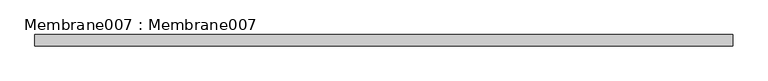
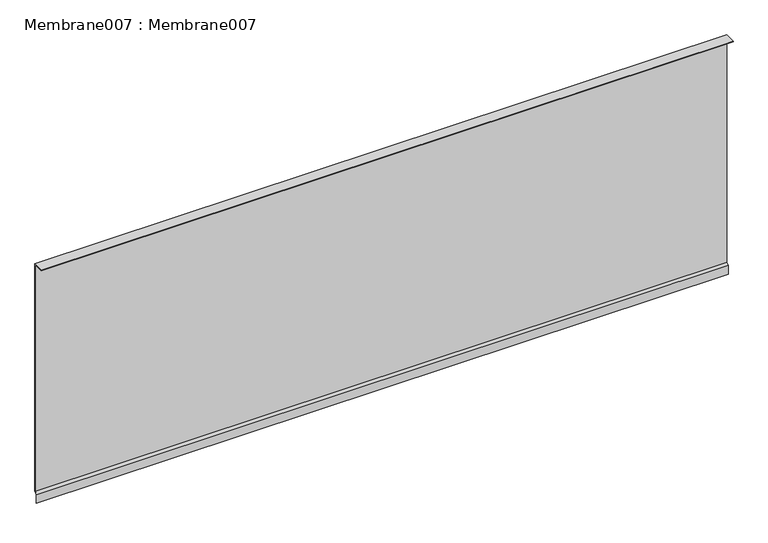
"""IFC4 building model written with IfcOpenShell, lengths in millimetres: proxy geometry, Membrane007 : Membrane007."""

import ifcopenshell
import ifcopenshell.guid

model = None  # the IFC model being written
_history = None  # IfcOwnerHistory: only IFC2X3 demands one
_inside = {}  # id of a spatial element -> (the spatial element, [elements in it])
_under = {}  # id of a project, library or spatial element -> (it, [spatial elements below it])
_declared = {}  # id of a project -> (the project, [libraries it declares])
_typed = {}  # id of a type object -> (the type object, [elements of that type])
_made_of = {}  # id of a material, layer set ... -> (it, [elements and type objects made of it])


def new_model(schema):
    """Start an empty IFC model of exactly this schema.

    Asked for "IFC4X3", IfcOpenShell would pick the latest addendum, in which some entities
    have other attributes; the version numbers below select the first issue.
    IFC2X3 requires an IfcOwnerHistory on every rooted entity: one is made here for all.
    """
    global model, _history
    if schema == "IFC4X3":
        model = ifcopenshell.file(schema_version=(4, 3, 0, 0))
    else:
        model = ifcopenshell.file(schema=schema)
    _inside.clear()
    _under.clear()
    _declared.clear()
    _typed.clear()
    _made_of.clear()
    _history = None
    if model.schema == "IFC2X3":
        org = make("IfcOrganization", Name="unknown")
        user = make(
            "IfcPersonAndOrganization",
            ThePerson=make("IfcPerson", FamilyName="unknown"),
            TheOrganization=org,
        )
        app = make(
            "IfcApplication",
            ApplicationDeveloper=org,
            Version="unknown",
            ApplicationFullName="unknown",
            ApplicationIdentifier="unknown",
        )
        _history = make(
            "IfcOwnerHistory",
            OwningUser=user,
            OwningApplication=app,
            ChangeAction="ADDED",
            CreationDate=0,
        )
    return model


def make(cls, **values):
    """One entity of the class cls with the attributes given. An attribute that is None is left unset."""
    return model.create_entity(
        cls, **{name: value for name, value in values.items() if value is not None}
    )


def rooted(cls, **values):
    """An entity with a GlobalId (a new one), such as an element, a storey or a relation."""
    return make(cls, GlobalId=ifcopenshell.guid.new(), OwnerHistory=_history, **values)


def si_unit(unit_type, name, prefix=None):
    """IfcSIUnit, for example si_unit("LENGTHUNIT", "METRE", prefix="MILLI")."""
    return make("IfcSIUnit", UnitType=unit_type, Prefix=prefix, Name=name)


def assignment(units):
    """IfcUnitAssignment: the units of a project."""
    return None if units is None else make("IfcUnitAssignment", Units=units)


def point(xyz):
    """IfcCartesianPoint."""
    return None if xyz is None else make("IfcCartesianPoint", Coordinates=xyz)


def direction(xyz):
    """IfcDirection."""
    return None if xyz is None else make("IfcDirection", DirectionRatios=xyz)


def frame(location, z_axis=None, x_axis=None):
    """IfcAxis2Placement3D, a coordinate frame: its origin and axes. An axis left out is left unset."""
    return make(
        "IfcAxis2Placement3D",
        Location=point(location),
        Axis=direction(z_axis),
        RefDirection=direction(x_axis),
    )


def origin():
    """The frame at (0, 0, 0) with its axes left unset."""
    return frame((0.0, 0.0, 0.0))


def place(relative_to, where):
    """IfcLocalPlacement: puts the frame where relative to a parent placement (None: the world)."""
    return make(
        "IfcLocalPlacement", PlacementRelTo=relative_to, RelativePlacement=where
    )


def context(
    kind, dimensions, precision=None, world=None, true_north=None, identifier=None
):
    """IfcGeometricRepresentationContext, for example the 3D "Model" context."""
    return make(
        "IfcGeometricRepresentationContext",
        ContextIdentifier=identifier,
        ContextType=kind,
        CoordinateSpaceDimension=dimensions,
        Precision=precision,
        WorldCoordinateSystem=world,
        TrueNorth=true_north,
    )


def project(units=None, contexts=None):
    """IfcProject with its units and contexts."""
    return rooted(
        "IfcProject",
        Name="project",
        RepresentationContexts=contexts,
        UnitsInContext=assignment(units),
    )


def spatial(cls, under=None, at=None, **own):
    """A site, building, storey or space (cls), placed at a placement, below another one or the project."""
    s = rooted(cls, ObjectPlacement=at, **own)
    if under is not None:
        _under.setdefault(under.id(), (under, []))[1].append(s)
    return s


def polyline(points):
    """IfcPolyline through the points."""
    return make("IfcPolyline", Points=[point(p) for p in points])


def outline(outer, holes=None, kind="AREA"):
    """IfcArbitraryClosedProfileDef: a profile drawn as a closed curve; with holes, ...WithVoids."""
    if holes is None:
        return make("IfcArbitraryClosedProfileDef", ProfileType=kind, OuterCurve=outer)
    return make(
        "IfcArbitraryProfileDefWithVoids",
        ProfileType=kind,
        OuterCurve=outer,
        InnerCurves=holes,
    )


def extrude(swept, where, along, depth):
    """IfcExtrudedAreaSolid: the profile swept, set in the frame where, extruded along a direction by depth."""
    return make(
        "IfcExtrudedAreaSolid",
        SweptArea=swept,
        Position=where,
        ExtrudedDirection=direction(along),
        Depth=depth,
    )


def shape(context_of_items, identifier, shape_type, items):
    """IfcShapeRepresentation: the items that make up one representation, for example the "Body"."""
    return make(
        "IfcShapeRepresentation",
        ContextOfItems=context_of_items,
        RepresentationIdentifier=identifier,
        RepresentationType=shape_type,
        Items=items,
    )


def source(mapping_origin, context_of_items, identifier, shape_type, items):
    """IfcRepresentationMap: a shape defined once, which mapped items show again and again."""
    return make(
        "IfcRepresentationMap",
        MappingOrigin=mapping_origin,
        MappedRepresentation=shape(context_of_items, identifier, shape_type, items),
    )


def transform(
    local_origin,
    x_axis=None,
    y_axis=None,
    z_axis=None,
    scale=None,
    scale2=None,
    scale3=None,
    uniform=True,
):
    """IfcCartesianTransformationOperator3D, or its non-uniform kind. x_axis, y_axis, z_axis: its Axis1, 2, 3."""
    if uniform:
        return make(
            "IfcCartesianTransformationOperator3D",
            Axis1=direction(x_axis),
            Axis2=direction(y_axis),
            LocalOrigin=point(local_origin),
            Scale=scale,
            Axis3=direction(z_axis),
        )
    return make(
        "IfcCartesianTransformationOperator3DnonUniform",
        Axis1=direction(x_axis),
        Axis2=direction(y_axis),
        LocalOrigin=point(local_origin),
        Scale=scale,
        Axis3=direction(z_axis),
        Scale2=scale2,
        Scale3=scale3,
    )


def mapped(mapping_source, mapping_target):
    """IfcMappedItem: shows the shape of a source again, moved by a transform."""
    return make(
        "IfcMappedItem", MappingSource=mapping_source, MappingTarget=mapping_target
    )


def made_of(thing, what):
    """Note that an element or type object is made of a material, layer set ...; save() writes the relation."""
    if what is not None:
        _made_of.setdefault(what.id(), (what, []))[1].append(thing)
    return thing


def element(
    cls,
    number,
    at=None,
    inside=None,
    cuts=None,
    type_object=None,
    material=None,
    context=None,
    identifier="Body",
    shape_type=None,
    held_by="IfcProductDefinitionShape",
    body=None,
    shapes=None,
    **own,
):
    """One element of the class cls, such as IfcWall. Its Tag is "e" and its number.

    at: its placement. inside: the storey or other place that contains it. cuts: it is an
    opening in that element (IfcRelVoidsElement). A single representation is given by context,
    identifier, shape_type and body (its items); several are given by shapes. held_by: the class
    of the entity that holds the representations. save() writes the other relations.
    """
    e = rooted(cls, Tag="e%d" % number, ObjectPlacement=at, **own)
    if body is not None:
        shapes = [shape(context, identifier, shape_type, body)]
    if shapes is not None:
        e.Representation = make(held_by, Representations=shapes)
    if inside is not None:
        _inside.setdefault(inside.id(), (inside, []))[1].append(e)
    if cuts is not None:
        rooted(
            "IfcRelVoidsElement", RelatingBuildingElement=cuts, RelatedOpeningElement=e
        )
    if type_object is not None:
        _typed.setdefault(type_object.id(), (type_object, []))[1].append(e)
    return made_of(e, material)


def aggregate(whole, parts):
    """IfcRelAggregates: a whole, such as a stair, and the parts it consists of."""
    return rooted("IfcRelAggregates", RelatingObject=whole, RelatedObjects=parts)


def save(model, path):
    """Write the relations noted so far, then the file.

    IfcRelAggregates (storeys below a building ...), IfcRelContainedInSpatialStructure (elements
    in a storey), IfcRelDefinesByType, IfcRelAssociatesMaterial and IfcRelDeclares: one each for
    every whole, place, type object, material and project.
    """
    for whole, parts in _under.values():
        aggregate(whole, parts)
    for where, things in _inside.values():
        rooted(
            "IfcRelContainedInSpatialStructure",
            RelatedElements=things,
            RelatingStructure=where,
        )
    for kind, things in _typed.values():
        rooted("IfcRelDefinesByType", RelatedObjects=things, RelatingType=kind)
    for what, things in _made_of.values():
        rooted("IfcRelAssociatesMaterial", RelatedObjects=things, RelatingMaterial=what)
    for by, libraries in _declared.values():
        rooted("IfcRelDeclares", RelatingContext=by, RelatedDefinitions=libraries)
    model.write(path)


def membrane007_membrane007_1038f70a(model_context):
    return source(origin(), model_context, "Body", "SweptSolid", [
        extrude(outline(polyline([(-4691.2641602, 39753.4375), (-4691.2641602, 39754.9375), (-4658.5039062, 39754.9375), (-4658.5039062, 39060.3828125), (-4664.7380371, 39054.1486816), (-4664.7380371, 39028.625), (-4666.2380371, 39028.625), (-4666.2380371, 39054.772171), (-4660.0039063, 39061.0063018), (-4660.0039063, 39753.4375), (-4691.2641602, 39753.4375)])), frame((12383.0178845, 0.0, 0.0), z_axis=(1.0, 0.0, 0.0), x_axis=(0.0, 1.0, 0.0)), (0.0, 0.0, 1.0), 2000.0),
    ])


if __name__ == "__main__":
    model = new_model("IFC4")
    model_context = context("Model", 3, world=origin())
    ifc_project = project(units=[si_unit("LENGTHUNIT", "METRE", prefix="MILLI")], contexts=[model_context])
    site = spatial("IfcSite", under=ifc_project)
    building = spatial("IfcBuilding", under=site)
    placement = place(None, origin())
    membrane007_membrane007_shape = membrane007_membrane007_1038f70a(model_context)
    element("IfcBuildingElementProxy", 1, Name="Membrane007 : Membrane007", ObjectType="Membrane007 : Membrane007", at=placement, inside=building, context=model_context, shape_type="MappedRepresentation", body=[
        mapped(membrane007_membrane007_shape, transform((0.0, 0.0, 0.0), x_axis=(1.0, 0.0, 0.0), y_axis=(0.0, 1.0, 0.0), z_axis=(0.0, 0.0, 1.0))),
    ])
    save(model, "model.ifc")

# Revit data of these elements
# Type "Membrane007 : Membrane007"
#   NameOverride = "Membrane007"
# Element 1 (IfcBuildingElementProxy, "Membrane007 : Membrane007")
#   Materials on its faces: "(2) LAYERS OF ICE & WATER SHIELD (BITUTHANE) UNDER STUCCO"
# Materials
#   "(2) LAYERS OF ICE & WATER SHIELD (BITUTHANE) UNDER STUCCO": class "Unassigned", colour RGB 186 255 159, transparency 0, Cost = 0
